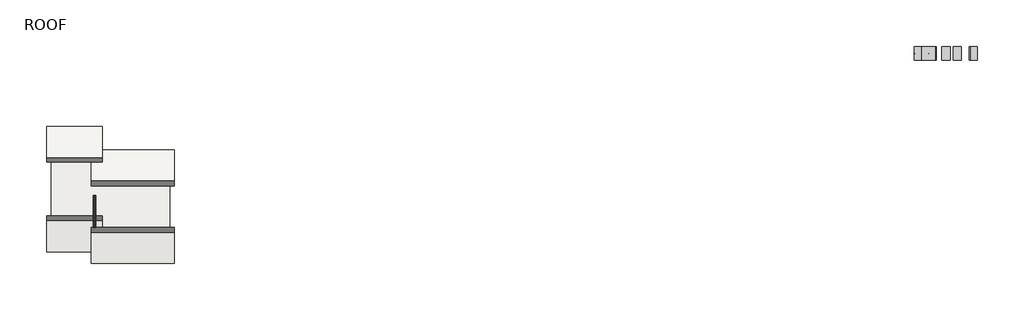
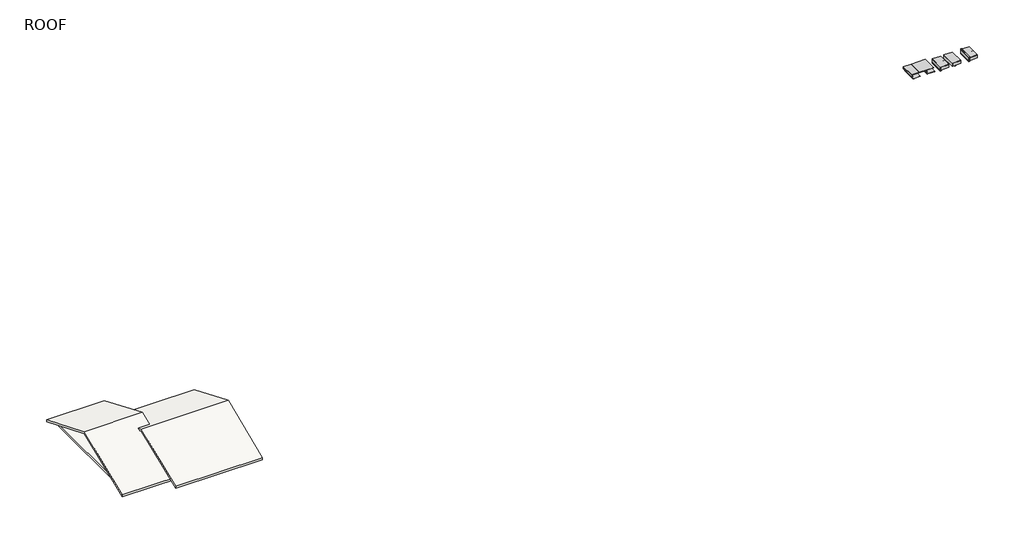
# One storey: 38 proxies, 2 roofs, 1 covering, 1 wall.
"""IFC4 building model written with IfcOpenShell, lengths in millimetres."""

import ifcopenshell
import ifcopenshell.guid

model = None  # the IFC model being written
_history = None  # IfcOwnerHistory: only IFC2X3 demands one
_inside = {}  # id of a spatial element -> (the spatial element, [elements in it])
_under = {}  # id of a project, library or spatial element -> (it, [spatial elements below it])
_declared = {}  # id of a project -> (the project, [libraries it declares])
_typed = {}  # id of a type object -> (the type object, [elements of that type])
_made_of = {}  # id of a material, layer set ... -> (it, [elements and type objects made of it])


def new_model(schema):
    """Start an empty IFC model of exactly this schema.

    Asked for "IFC4X3", IfcOpenShell would pick the latest addendum, in which some entities
    have other attributes; the version numbers below select the first issue.
    IFC2X3 requires an IfcOwnerHistory on every rooted entity: one is made here for all.
    """
    global model, _history
    if schema == "IFC4X3":
        model = ifcopenshell.file(schema_version=(4, 3, 0, 0))
    else:
        model = ifcopenshell.file(schema=schema)
    _inside.clear()
    _under.clear()
    _declared.clear()
    _typed.clear()
    _made_of.clear()
    _history = None
    if model.schema == "IFC2X3":
        org = make("IfcOrganization", Name="unknown")
        user = make(
            "IfcPersonAndOrganization",
            ThePerson=make("IfcPerson", FamilyName="unknown"),
            TheOrganization=org,
        )
        app = make(
            "IfcApplication",
            ApplicationDeveloper=org,
            Version="unknown",
            ApplicationFullName="unknown",
            ApplicationIdentifier="unknown",
        )
        _history = make(
            "IfcOwnerHistory",
            OwningUser=user,
            OwningApplication=app,
            ChangeAction="ADDED",
            CreationDate=0,
        )
    return model


def make(cls, **values):
    """One entity of the class cls with the attributes given. An attribute that is None is left unset."""
    return model.create_entity(
        cls, **{name: value for name, value in values.items() if value is not None}
    )


def rooted(cls, **values):
    """An entity with a GlobalId (a new one), such as an element, a storey or a relation."""
    return make(cls, GlobalId=ifcopenshell.guid.new(), OwnerHistory=_history, **values)


def si_unit(unit_type, name, prefix=None):
    """IfcSIUnit, for example si_unit("LENGTHUNIT", "METRE", prefix="MILLI")."""
    return make("IfcSIUnit", UnitType=unit_type, Prefix=prefix, Name=name)


def assignment(units):
    """IfcUnitAssignment: the units of a project."""
    return None if units is None else make("IfcUnitAssignment", Units=units)


def point(xyz):
    """IfcCartesianPoint."""
    return None if xyz is None else make("IfcCartesianPoint", Coordinates=xyz)


def direction(xyz):
    """IfcDirection."""
    return None if xyz is None else make("IfcDirection", DirectionRatios=xyz)


def frame(location, z_axis=None, x_axis=None):
    """IfcAxis2Placement3D, a coordinate frame: its origin and axes. An axis left out is left unset."""
    return make(
        "IfcAxis2Placement3D",
        Location=point(location),
        Axis=direction(z_axis),
        RefDirection=direction(x_axis),
    )


def origin():
    """The frame at (0, 0, 0) with its axes left unset."""
    return frame((0.0, 0.0, 0.0))


def place(relative_to, where):
    """IfcLocalPlacement: puts the frame where relative to a parent placement (None: the world)."""
    return make(
        "IfcLocalPlacement", PlacementRelTo=relative_to, RelativePlacement=where
    )


def context(
    kind, dimensions, precision=None, world=None, true_north=None, identifier=None
):
    """IfcGeometricRepresentationContext, for example the 3D "Model" context."""
    return make(
        "IfcGeometricRepresentationContext",
        ContextIdentifier=identifier,
        ContextType=kind,
        CoordinateSpaceDimension=dimensions,
        Precision=precision,
        WorldCoordinateSystem=world,
        TrueNorth=true_north,
    )


def project(units=None, contexts=None):
    """IfcProject with its units and contexts."""
    return rooted(
        "IfcProject",
        Name="project",
        RepresentationContexts=contexts,
        UnitsInContext=assignment(units),
    )


def spatial(cls, under=None, at=None, **own):
    """A site, building, storey or space (cls), placed at a placement, below another one or the project."""
    s = rooted(cls, ObjectPlacement=at, **own)
    if under is not None:
        _under.setdefault(under.id(), (under, []))[1].append(s)
    return s


def polyline(points):
    """IfcPolyline through the points."""
    return make("IfcPolyline", Points=[point(p) for p in points])


def outline(outer, holes=None, kind="AREA"):
    """IfcArbitraryClosedProfileDef: a profile drawn as a closed curve; with holes, ...WithVoids."""
    if holes is None:
        return make("IfcArbitraryClosedProfileDef", ProfileType=kind, OuterCurve=outer)
    return make(
        "IfcArbitraryProfileDefWithVoids",
        ProfileType=kind,
        OuterCurve=outer,
        InnerCurves=holes,
    )


def extrude(swept, where, along, depth):
    """IfcExtrudedAreaSolid: the profile swept, set in the frame where, extruded along a direction by depth."""
    return make(
        "IfcExtrudedAreaSolid",
        SweptArea=swept,
        Position=where,
        ExtrudedDirection=direction(along),
        Depth=depth,
    )


def faces_of(points, faces, orient=None, outer=None):
    """IfcFace entities. A face is a list of loops; a loop is a list of indices into points, from 0.

    orient and outer hold one flag for each loop. By default every Orientation is true, the
    first loop of a face is its IfcFaceOuterBound and the others are IfcFaceBound.
    """
    made = []
    for i, loops in enumerate(faces):
        bounds = []
        for j, loop in enumerate(loops):
            is_outer = j == 0 if outer is None else outer[i][j]
            bounds.append(
                make(
                    "IfcFaceOuterBound" if is_outer else "IfcFaceBound",
                    Bound=make("IfcPolyLoop", Polygon=[points[k] for k in loop]),
                    Orientation=True if orient is None else orient[i][j],
                )
            )
        made.append(make("IfcFace", Bounds=bounds))
    return made


def faceted_brep(points, faces, orient=None, outer=None, voids=None):
    """IfcFacetedBrep: a solid bounded by flat faces; with voids (closed shells), ...WithVoids."""
    shared = [point(p) for p in points]
    hull = make("IfcClosedShell", CfsFaces=faces_of(shared, faces, orient, outer))
    if voids is None:
        return make("IfcFacetedBrep", Outer=hull)
    return make(
        "IfcFacetedBrepWithVoids",
        Outer=hull,
        Voids=[
            make(cls, CfsFaces=faces_of(shared, fs, o, b)) for cls, fs, o, b in voids
        ],
    )


def shape(context_of_items, identifier, shape_type, items):
    """IfcShapeRepresentation: the items that make up one representation, for example the "Body"."""
    return make(
        "IfcShapeRepresentation",
        ContextOfItems=context_of_items,
        RepresentationIdentifier=identifier,
        RepresentationType=shape_type,
        Items=items,
    )


def source(mapping_origin, context_of_items, identifier, shape_type, items):
    """IfcRepresentationMap: a shape defined once, which mapped items show again and again."""
    return make(
        "IfcRepresentationMap",
        MappingOrigin=mapping_origin,
        MappedRepresentation=shape(context_of_items, identifier, shape_type, items),
    )


def transform(
    local_origin,
    x_axis=None,
    y_axis=None,
    z_axis=None,
    scale=None,
    scale2=None,
    scale3=None,
    uniform=True,
):
    """IfcCartesianTransformationOperator3D, or its non-uniform kind. x_axis, y_axis, z_axis: its Axis1, 2, 3."""
    if uniform:
        return make(
            "IfcCartesianTransformationOperator3D",
            Axis1=direction(x_axis),
            Axis2=direction(y_axis),
            LocalOrigin=point(local_origin),
            Scale=scale,
            Axis3=direction(z_axis),
        )
    return make(
        "IfcCartesianTransformationOperator3DnonUniform",
        Axis1=direction(x_axis),
        Axis2=direction(y_axis),
        LocalOrigin=point(local_origin),
        Scale=scale,
        Axis3=direction(z_axis),
        Scale2=scale2,
        Scale3=scale3,
    )


def mapped(mapping_source, mapping_target):
    """IfcMappedItem: shows the shape of a source again, moved by a transform."""
    return make(
        "IfcMappedItem", MappingSource=mapping_source, MappingTarget=mapping_target
    )


def made_of(thing, what):
    """Note that an element or type object is made of a material, layer set ...; save() writes the relation."""
    if what is not None:
        _made_of.setdefault(what.id(), (what, []))[1].append(thing)
    return thing


def element(
    cls,
    number,
    at=None,
    inside=None,
    cuts=None,
    type_object=None,
    material=None,
    context=None,
    identifier="Body",
    shape_type=None,
    held_by="IfcProductDefinitionShape",
    body=None,
    shapes=None,
    **own,
):
    """One element of the class cls, such as IfcWall. Its Tag is "e" and its number.

    at: its placement. inside: the storey or other place that contains it. cuts: it is an
    opening in that element (IfcRelVoidsElement). A single representation is given by context,
    identifier, shape_type and body (its items); several are given by shapes. held_by: the class
    of the entity that holds the representations. save() writes the other relations.
    """
    e = rooted(cls, Tag="e%d" % number, ObjectPlacement=at, **own)
    if body is not None:
        shapes = [shape(context, identifier, shape_type, body)]
    if shapes is not None:
        e.Representation = make(held_by, Representations=shapes)
    if inside is not None:
        _inside.setdefault(inside.id(), (inside, []))[1].append(e)
    if cuts is not None:
        rooted(
            "IfcRelVoidsElement", RelatingBuildingElement=cuts, RelatedOpeningElement=e
        )
    if type_object is not None:
        _typed.setdefault(type_object.id(), (type_object, []))[1].append(e)
    return made_of(e, material)


def aggregate(whole, parts):
    """IfcRelAggregates: a whole, such as a stair, and the parts it consists of."""
    return rooted("IfcRelAggregates", RelatingObject=whole, RelatedObjects=parts)


def save(model, path):
    """Write the relations noted so far, then the file.

    IfcRelAggregates (storeys below a building ...), IfcRelContainedInSpatialStructure (elements
    in a storey), IfcRelDefinesByType, IfcRelAssociatesMaterial and IfcRelDeclares: one each for
    every whole, place, type object, material and project.
    """
    for whole, parts in _under.values():
        aggregate(whole, parts)
    for where, things in _inside.values():
        rooted(
            "IfcRelContainedInSpatialStructure",
            RelatedElements=things,
            RelatingStructure=where,
        )
    for kind, things in _typed.values():
        rooted("IfcRelDefinesByType", RelatedObjects=things, RelatingType=kind)
    for what, things in _made_of.values():
        rooted("IfcRelAssociatesMaterial", RelatedObjects=things, RelatingMaterial=what)
    for by, libraries in _declared.values():
        rooted("IfcRelDeclares", RelatingContext=by, RelatedDefinitions=libraries)
    model.write(path)


def generic_models_10_generic_models_1_ea081297(model_context):
    return source(origin(), model_context, "Body", "SweptSolid", [
        extrude(outline(polyline([(49758.6, 0.0), (49720.5, 0.0), (49720.5, 1219.2), (49758.6, 1219.2), (49758.6, 0.0)])), frame((0.0, 0.0, 5507.83125), z_axis=(0.0, 0.0, 1.0), x_axis=(1.0, 0.0, 0.0)), (0.0, 0.0, 1.0), 139.7),
    ])


def generic_models_109_generic_models_1_8619d77b(model_context):
    return source(origin(), model_context, "Body", "SweptSolid", [
        extrude(outline(polyline([(51003.2, 0.0), (50914.3, 0.0), (50914.3, 1219.2), (51003.2, 1219.2), (51003.2, 0.0)])), frame((0.0, 0.0, 5184.378125), z_axis=(0.0, 0.0, 1.0), x_axis=(1.0, 0.0, 0.0)), (0.0, 0.0, 1.0), 38.1),
    ])


def generic_models_110_generic_models_1_6bdce9b6(model_context):
    return source(origin(), model_context, "Body", "SweptSolid", [
        extrude(outline(polyline([(51642.1451407, 1219.2), (51642.1451407, 0.0), (50914.3, 0.0), (50914.3, 1219.2), (51642.1451407, 1219.2)])), frame((0.0, 0.0, 5508.228125), z_axis=(0.0, 0.0, 1.0), x_axis=(1.0, 0.0, 0.0)), (0.0, 0.0, 1.0), 19.05),
    ])


def generic_models_112_generic_models_65_d168d7b0(model_context):
    return source(origin(), model_context, "Body", "SweptSolid", [
        extrude(outline(polyline([(50952.4, 592.1375), (50952.4, 630.2375), (51642.1451407, 630.2375), (51642.1451407, 592.1375), (50952.4, 592.1375)])), frame((0.0, 0.0, 5222.478125), z_axis=(0.0, 0.0, 1.0), x_axis=(1.0, 0.0, 0.0)), (0.0, 0.0, 1.0), 285.75),
    ])


def generic_models_113_generic_models_1_101608ab(model_context):
    return source(origin(), model_context, "Body", "SweptSolid", [
        extrude(outline(polyline([(52171.6, 0.0), (52133.5, 0.0), (52133.5, 1219.2), (52171.6, 1219.2), (52171.6, 0.0)])), frame((0.0, 0.0, 5222.478125), z_axis=(0.0, 0.0, 1.0), x_axis=(1.0, 0.0, 0.0)), (0.0, 0.0, 1.0), 285.75),
    ])


def generic_models_114_generic_models_1_a6fb1c2c(model_context):
    return source(origin(), model_context, "Body", "SweptSolid", [
        extrude(outline(polyline([(51642.1451407, 1219.2), (51642.1451407, 0.0), (50965.9242022, 0.0), (50965.9242022, 1219.2), (51642.1451407, 1219.2)])), frame((0.0, 0.0, 5237.6235034), z_axis=(0.0, 0.0, 1.0), x_axis=(1.0, 0.0, 0.0)), (0.0, 0.0, 1.0), 254.0),
    ])


def generic_models_12_generic_models_46_b8a9a4e8(model_context):
    return source(origin(), model_context, "Body", "SweptSolid", [
        extrude(outline(polyline([(49757.8505137, 0.0), (49721.1284797, 0.0), (49721.1284797, 1219.2), (49757.8505137, 1219.2), (49757.8505137, 0.0)])), frame((0.0, 0.0, 5505.7509163), z_axis=(0.0, 0.0, 1.0), x_axis=(1.0, 0.0, 0.0)), (0.0, 0.0, 1.0), 1.5875),
    ])


def generic_models_13_generic_models_65_9e643fb9(model_context):
    return source(origin(), model_context, "Body", "SweptSolid", [
        extrude(outline(polyline([(49128.3625, 592.1375), (49128.3625, 630.2375), (50347.5625, 630.2375), (50347.5625, 592.1375), (49128.3625, 592.1375)])), frame((0.0, 0.0, 5507.83125), z_axis=(0.0, 0.0, 1.0), x_axis=(1.0, 0.0, 0.0)), (0.0, 0.0, 1.0), 139.7),
    ])


def generic_models_14_generic_models_1_e8c90d4c(model_context):
    return source(origin(), model_context, "Body", "SweptSolid", [
        extrude(outline(polyline([(2277.1204978, 49799.875), (2239.0204978, 49799.875), (2239.0204978, 49825.275), (2240.6079978, 49825.275), (2240.6079978, 49801.4625), (2277.1204978, 49801.4625), (2277.1204978, 49799.875)])), frame((0.0, 0.0, 0.0), z_axis=(0.0, 1.0, 0.0), x_axis=(0.0, 0.0, 1.0)), (0.0, 0.0, 1.0), 1219.2),
    ])


def generic_models_22_generic_models_1_e5767157(model_context):
    return source(origin(), model_context, "Body", "SweptSolid", [
        extrude(outline(polyline([(2409.6091, 49800.66875), (2409.6091, 49799.875), (2407.0592364, 49799.875), (2405.4618473, 49749.075), (2404.6631527, 49749.075), (2403.0657636, 49799.875), (2400.5159, 49799.875), (2400.5159, 49800.66875), (2409.6091, 49800.66875)])), frame((0.0, 565.15, 0.0), z_axis=(0.0, 1.0, 0.0), x_axis=(0.0, 0.0, 1.0)), (0.0, 0.0, 1.0), 12.7),
    ])


def generic_models_226_generic_models_1_7dc37832(model_context):
    return source(origin(), model_context, "Body", "SweptSolid", [
        extrude(outline(polyline([(5263.35625, 49733.4159), (5263.35625, 49742.5091), (5264.15, 49742.5091), (5264.15, 49739.9592364), (5314.95, 49738.3618473), (5314.95, 49737.5631527), (5264.15, 49735.9657636), (5264.15, 49733.4159), (5263.35625, 49733.4159)])), frame((0.0, 565.15, 0.0), z_axis=(0.0, 1.0, 0.0), x_axis=(0.0, 0.0, 1.0)), (0.0, 0.0, 1.0), 12.7),
    ])


def generic_models_202_generic_models_1_0ad20a8b(model_context):
    return source(origin(), model_context, "Body", "SweptSolid", [
        extrude(outline(polyline([(2253.330428, 49813.3451407), (2242.217928, 49813.3451407), (2242.217928, 49826.0451407), (2234.280428, 49828.9341545), (2234.280428, 50422.9451407), (2253.330428, 50422.9451407), (2253.330428, 49813.3451407)])), frame((0.0, 0.0, 0.0), z_axis=(0.0, 1.0, 0.0), x_axis=(0.0, 0.0, 1.0)), (0.0, 0.0, 1.0), 1219.2),
    ])


def generic_models_233_generic_models_1_ae5bae41(model_context):
    return source(origin(), model_context, "Body", "SweptSolid", [
        extrude(outline(polyline([(48564.8, 0.0), (48475.9, 0.0), (48475.9, 1219.2), (48564.8, 1219.2), (48564.8, 0.0)])), frame((0.0, 0.0, 5467.35), z_axis=(0.0, 0.0, 1.0), x_axis=(1.0, 0.0, 0.0)), (0.0, 0.0, 1.0), 38.1),
    ])


def generic_models_236_generic_models_1_f8917e71(model_context):
    return source(origin(), model_context, "Body", "SweptSolid", [
        extrude(outline(polyline([(48507.65, 0.0), (48469.55, 0.0), (48469.55, 1219.2), (48507.65, 1219.2), (48507.65, 0.0)])), frame((0.0, 0.0, 5507.83125), z_axis=(0.0, 0.0, 1.0), x_axis=(1.0, 0.0, 0.0)), (0.0, 0.0, 1.0), 139.7),
    ])


def generic_models_237_generic_models_65_1df05f16(model_context):
    return source(origin(), model_context, "Body", "SweptSolid", [
        extrude(outline(polyline([(48469.55, 592.1375), (48469.55, 630.2375), (49128.3625, 630.2375), (49128.3625, 592.1375), (48469.55, 592.1375)])), frame((0.0, 0.0, 5507.83125), z_axis=(0.0, 0.0, 1.0), x_axis=(1.0, 0.0, 0.0)), (0.0, 0.0, 1.0), 139.7),
    ])


def generic_models_239_generic_models_46_95e6735a(model_context):
    return source(origin(), model_context, "Body", "SweptSolid", [
        extrude(outline(polyline([(50347.5625, 0.0), (49691.4320511, 0.0), (49691.4320511, 1219.2), (50347.5625, 1219.2), (50347.5625, 0.0)])), frame((0.0, 0.0, 5505.7509163), z_axis=(0.0, 0.0, 1.0), x_axis=(1.0, 0.0, 0.0)), (0.0, 0.0, 1.0), 1.5875),
    ])


def generic_models_240_generic_models_1_611786cf(model_context):
    return source(origin(), model_context, "Body", "SweptSolid", [
        extrude(outline(polyline([(49128.3625, 1219.2), (49128.3625, 0.0), (48469.55, 0.0), (48469.55, 1219.2), (49128.3625, 1219.2)])), frame((0.0, 0.0, 5649.9125), z_axis=(0.0, 0.0, 1.0), x_axis=(1.0, 0.0, 0.0)), (0.0, 0.0, 1.0), 19.05),
    ])


def generic_models_29_generic_models_1_59087225(model_context):
    return source(origin(), model_context, "Body", "SweptSolid", [
        extrude(outline(polyline([(50347.5625, 1219.2), (50347.5625, 0.0), (49128.3625, 0.0), (49128.3625, 1219.2), (50347.5625, 1219.2)])), frame((0.0, 0.0, 5647.53125), z_axis=(0.0, 0.0, 1.0), x_axis=(1.0, 0.0, 0.0)), (0.0, 0.0, 1.0), 19.05),
    ])


def generic_models_37_generic_models_1_916dd7c6(model_context):
    return source(origin(), model_context, "Body", "SweptSolid", [
        extrude(outline(polyline([(2409.6091, 49675.25625), (2400.5159, 49675.25625), (2400.5159, 49676.05), (2403.0657636, 49676.05), (2404.6631527, 49726.85), (2405.4618473, 49726.85), (2407.0592364, 49676.05), (2409.6091, 49676.05), (2409.6091, 49675.25625)])), frame((0.0, 565.15, 0.0), z_axis=(0.0, 1.0, 0.0), x_axis=(0.0, 0.0, 1.0)), (0.0, 0.0, 1.0), 12.7),
    ])


def generic_models_103_generic_models_1_250a6a11(model_context):
    return source(origin(), model_context, "Body", "SweptSolid", [
        extrude(outline(polyline([(49784.0, 0.0), (49695.1, 0.0), (49695.1, 1219.2), (49784.0, 1219.2), (49784.0, 0.0)])), frame((0.0, 0.0, 5264.15), z_axis=(0.0, 0.0, 1.0), x_axis=(1.0, 0.0, 0.0)), (0.0, 0.0, 1.0), 38.1),
    ])


def generic_models_71_generic_models_1_508a995f(model_context):
    return source(origin(), model_context, "Body", "SweptSolid", [
        extrude(outline(polyline([(50952.4, 0.0), (50914.3, 0.0), (50914.3, 1219.2), (50952.4, 1219.2), (50952.4, 0.0)])), frame((0.0, 0.0, 5222.478125), z_axis=(0.0, 0.0, 1.0), x_axis=(1.0, 0.0, 0.0)), (0.0, 0.0, 1.0), 285.75),
    ])


def generic_models_87_generic_models_1_55a64953(model_context):
    return source(origin(), model_context, "Body", "SweptSolid", [
        extrude(outline(polyline([(51968.4, 0.0), (51930.3, 0.0), (51930.3, 1219.2), (51968.4, 1219.2), (51968.4, 0.0)])), frame((0.0, 0.0, 5222.478125), z_axis=(0.0, 0.0, 1.0), x_axis=(1.0, 0.0, 0.0)), (0.0, 0.0, 1.0), 285.75),
    ])


model = new_model("IFC4")

# Units and contexts
model_context = context("Model", 3, world=origin())
ifc_project = project(units=[si_unit("LENGTHUNIT", "METRE", prefix="MILLI")], contexts=[model_context])

# Site, building, storey
site = spatial("IfcSite", under=ifc_project)
building = spatial("IfcBuilding", under=site)
storey = spatial("IfcBuildingStorey", under=building, Name="ROOF", Elevation=5130.8)

# Proxies
placement = place(None, origin())
generic_models_10_generic_models_1_shape = generic_models_10_generic_models_1_ea081297(model_context)
element("IfcBuildingElementProxy", 1, Name="Generic Models 10 : Generic Models 1", ObjectType="Generic Models 10 : Generic Models 1", at=placement, inside=storey, context=model_context, shape_type="MappedRepresentation", body=[
    mapped(generic_models_10_generic_models_1_shape, transform((0.0, 0.0, 0.0), x_axis=(1.0, 0.0, 0.0), y_axis=(0.0, 1.0, 0.0), z_axis=(0.0, 0.0, 1.0))),
])
generic_models_109_generic_models_1_shape = generic_models_109_generic_models_1_8619d77b(model_context)
element("IfcBuildingElementProxy", 2, Name="Generic Models 109 : Generic Models 1", ObjectType="Generic Models 109 : Generic Models 1", at=placement, inside=storey, context=model_context, shape_type="MappedRepresentation", body=[
    mapped(generic_models_109_generic_models_1_shape, transform((2438.4, 0.0, 0.0), x_axis=(1.0, 0.0, 0.0), y_axis=(0.0, 1.0, 0.0), z_axis=(0.0, 0.0, 1.0))),
])
generic_models_110_generic_models_1_shape = generic_models_110_generic_models_1_6bdce9b6(model_context)
element("IfcBuildingElementProxy", 3, Name="Generic Models 110 : Generic Models 1", ObjectType="Generic Models 110 : Generic Models 1", at=placement, inside=storey, context=model_context, shape_type="MappedRepresentation", body=[
    mapped(generic_models_110_generic_models_1_shape, transform((2438.4, 0.0, 0.0), x_axis=(1.0, 0.0, 0.0), y_axis=(0.0, 1.0, 0.0), z_axis=(0.0, 0.0, 1.0))),
])
element("IfcBuildingElementProxy", 4, Name="Generic Models 111 : Generic Models 1", ObjectType="Generic Models 111 : Generic Models 1", at=placement, inside=storey, context=model_context, shape_type="MappedRepresentation", body=[
    mapped(generic_models_109_generic_models_1_shape, transform((2438.4, 0.0, -38.1), x_axis=(1.0, 0.0, 0.0), y_axis=(0.0, 1.0, 0.0), z_axis=(0.0, 0.0, 1.0))),
])
generic_models_112_generic_models_65_shape = generic_models_112_generic_models_65_d168d7b0(model_context)
element("IfcBuildingElementProxy", 5, Name="Generic Models 112 : Generic Models 65", ObjectType="Generic Models 112 : Generic Models 65", at=placement, inside=storey, context=model_context, shape_type="MappedRepresentation", body=[
    mapped(generic_models_112_generic_models_65_shape, transform((2438.4, 0.0, 0.0), x_axis=(1.0, 0.0, 0.0), y_axis=(0.0, 1.0, 0.0), z_axis=(0.0, 0.0, 1.0))),
])
generic_models_113_generic_models_1_shape = generic_models_113_generic_models_1_101608ab(model_context)
element("IfcBuildingElementProxy", 6, Name="Generic Models 113 : Generic Models 1", ObjectType="Generic Models 113 : Generic Models 1", at=placement, inside=storey, context=model_context, shape_type="MappedRepresentation", body=[
    mapped(generic_models_113_generic_models_1_shape, transform((1219.2, 0.0, 0.0), x_axis=(1.0, 0.0, 0.0), y_axis=(0.0, 1.0, 0.0), z_axis=(0.0, 0.0, 1.0))),
])
generic_models_114_generic_models_1_shape = generic_models_114_generic_models_1_a6fb1c2c(model_context)
element("IfcBuildingElementProxy", 7, Name="Generic Models 114 : Generic Models 1", ObjectType="Generic Models 114 : Generic Models 1", at=placement, inside=storey, context=model_context, shape_type="MappedRepresentation", body=[
    mapped(generic_models_114_generic_models_1_shape, transform((2438.4, 0.0, 0.0), x_axis=(1.0, 0.0, 0.0), y_axis=(0.0, 1.0, 0.0), z_axis=(0.0, 0.0, 1.0))),
])
element("IfcBuildingElementProxy", 8, Name="Generic Models 115 : Generic Models 1", ObjectType="Generic Models 115 : Generic Models 1", at=placement, inside=storey, context=model_context, shape_type="MappedRepresentation", body=[
    mapped(generic_models_109_generic_models_1_shape, transform((2438.4, 0.0, 342.9), x_axis=(1.0, 0.0, 0.0), y_axis=(0.0, 1.0, 0.0), z_axis=(0.0, 0.0, 1.0))),
])
generic_models_12_generic_models_46_shape = generic_models_12_generic_models_46_b8a9a4e8(model_context)
element("IfcBuildingElementProxy", 9, Name="Generic Models 12 : Generic Models 46", ObjectType="Generic Models 12 : Generic Models 46", at=placement, inside=storey, context=model_context, shape_type="MappedRepresentation", body=[
    mapped(generic_models_12_generic_models_46_shape, transform((0.0, 0.0, 0.0), x_axis=(1.0, 0.0, 0.0), y_axis=(0.0, 1.0, 0.0), z_axis=(0.0, 0.0, 1.0))),
])
generic_models_13_generic_models_65_shape = generic_models_13_generic_models_65_9e643fb9(model_context)
element("IfcBuildingElementProxy", 10, Name="Generic Models 13 : Generic Models 65", ObjectType="Generic Models 13 : Generic Models 65", at=placement, inside=storey, context=model_context, shape_type="MappedRepresentation", body=[
    mapped(generic_models_13_generic_models_65_shape, transform((0.0, 0.0, 0.0), x_axis=(1.0, 0.0, 0.0), y_axis=(0.0, 1.0, 0.0), z_axis=(0.0, 0.0, 1.0))),
])
generic_models_14_generic_models_1_shape = generic_models_14_generic_models_1_e8c90d4c(model_context)
element("IfcBuildingElementProxy", 11, Name="Generic Models 14 : Generic Models 1", ObjectType="Generic Models 14 : Generic Models 1", at=placement, inside=storey, context=model_context, shape_type="MappedRepresentation", body=[
    mapped(generic_models_14_generic_models_1_shape, transform((0.0, 0.0, 3050.778125), x_axis=(1.0, 0.0, 0.0), y_axis=(0.0, 1.0, 0.0), z_axis=(0.0, 0.0, 1.0))),
])
generic_models_22_generic_models_1_shape = generic_models_22_generic_models_1_e5767157(model_context)
element("IfcBuildingElementProxy", 12, Name="Generic Models 22 : Generic Models 1", ObjectType="Generic Models 22 : Generic Models 1", at=placement, inside=storey, context=model_context, shape_type="MappedRepresentation", body=[
    mapped(generic_models_22_generic_models_1_shape, transform((0.0, 0.0, 3081.3375), x_axis=(1.0, 0.0, 0.0), y_axis=(0.0, 1.0, 0.0), z_axis=(0.0, 0.0, 1.0))),
])
element("IfcBuildingElementProxy", 13, Name="Generic Models 224 : Generic Models 1", ObjectType="Generic Models 224 : Generic Models 1", at=placement, inside=storey, context=model_context, shape_type="MappedRepresentation", body=[
    mapped(generic_models_14_generic_models_1_shape, transform((-1217.6125, 0.0, 3050.778125), x_axis=(1.0, 0.0, 0.0), y_axis=(0.0, 1.0, 0.0), z_axis=(0.0, 0.0, 1.0))),
])
element("IfcBuildingElementProxy", 14, Name="Generic Models 225 : Generic Models 1", ObjectType="Generic Models 225 : Generic Models 1", at=placement, inside=storey, context=model_context, shape_type="MappedRepresentation", body=[
    mapped(generic_models_22_generic_models_1_shape, transform((-1219.2, 0.0, 3081.3375), x_axis=(1.0, 0.0, 0.0), y_axis=(0.0, 1.0, 0.0), z_axis=(0.0, 0.0, 1.0))),
])
generic_models_226_generic_models_1_shape = generic_models_226_generic_models_1_7dc37832(model_context)
element("IfcBuildingElementProxy", 15, Name="Generic Models 226 : Generic Models 1", ObjectType="Generic Models 226 : Generic Models 1", at=placement, inside=storey, context=model_context, shape_type="MappedRepresentation", body=[
    mapped(generic_models_226_generic_models_1_shape, transform((-1219.2, 0.0, 203.2), x_axis=(1.0, 0.0, 0.0), y_axis=(0.0, 1.0, 0.0), z_axis=(0.0, 0.0, 1.0))),
])
generic_models_202_generic_models_1_shape = generic_models_202_generic_models_1_0ad20a8b(model_context)
element("IfcBuildingElementProxy", 16, Name="Generic Models 231 : Generic Models 1", ObjectType="Generic Models 231 : Generic Models 1", at=placement, inside=storey, context=model_context, shape_type="MappedRepresentation", body=[
    mapped(generic_models_202_generic_models_1_shape, transform((-1217.6125, 0.0, 3050.778125), x_axis=(1.0, 0.0, 0.0), y_axis=(0.0, 1.0, 0.0), z_axis=(0.0, 0.0, 1.0))),
])
generic_models_233_generic_models_1_shape = generic_models_233_generic_models_1_ae5bae41(model_context)
element("IfcBuildingElementProxy", 17, Name="Generic Models 233 : Generic Models 1", ObjectType="Generic Models 233 : Generic Models 1", at=placement, inside=storey, context=model_context, shape_type="MappedRepresentation", body=[
    mapped(generic_models_233_generic_models_1_shape, transform((0.0, 0.0, 0.0), x_axis=(1.0, 0.0, 0.0), y_axis=(0.0, 1.0, 0.0), z_axis=(0.0, 0.0, 1.0))),
])
generic_models_236_generic_models_1_shape = generic_models_236_generic_models_1_f8917e71(model_context)
element("IfcBuildingElementProxy", 18, Name="Generic Models 236 : Generic Models 1", ObjectType="Generic Models 236 : Generic Models 1", at=placement, inside=storey, context=model_context, shape_type="MappedRepresentation", body=[
    mapped(generic_models_236_generic_models_1_shape, transform((0.0, 0.0, 0.0), x_axis=(1.0, 0.0, 0.0), y_axis=(0.0, 1.0, 0.0), z_axis=(0.0, 0.0, 1.0))),
])
generic_models_237_generic_models_65_shape = generic_models_237_generic_models_65_1df05f16(model_context)
element("IfcBuildingElementProxy", 19, Name="Generic Models 237 : Generic Models 65", ObjectType="Generic Models 237 : Generic Models 65", at=placement, inside=storey, context=model_context, shape_type="MappedRepresentation", body=[
    mapped(generic_models_237_generic_models_65_shape, transform((0.0, 0.0, 0.0), x_axis=(1.0, 0.0, 0.0), y_axis=(0.0, 1.0, 0.0), z_axis=(0.0, 0.0, 1.0))),
])
generic_models_239_generic_models_46_shape = generic_models_239_generic_models_46_95e6735a(model_context)
element("IfcBuildingElementProxy", 20, Name="Generic Models 239 : Generic Models 46", ObjectType="Generic Models 239 : Generic Models 46", at=placement, inside=storey, context=model_context, shape_type="MappedRepresentation", body=[
    mapped(generic_models_239_generic_models_46_shape, transform((-1219.2, 0.0, 142.08125), x_axis=(1.0, 0.0, 0.0), y_axis=(0.0, 1.0, 0.0), z_axis=(0.0, 0.0, 1.0))),
])
generic_models_240_generic_models_1_shape = generic_models_240_generic_models_1_611786cf(model_context)
element("IfcBuildingElementProxy", 21, Name="Generic Models 240 : Generic Models 1", ObjectType="Generic Models 240 : Generic Models 1", at=placement, inside=storey, context=model_context, shape_type="MappedRepresentation", body=[
    mapped(generic_models_240_generic_models_1_shape, transform((0.0, 0.0, 0.0), x_axis=(1.0, 0.0, 0.0), y_axis=(0.0, 1.0, 0.0), z_axis=(0.0, 0.0, 1.0))),
])
element("IfcBuildingElementProxy", 22, Name="Generic Models 25 : Generic Models 46", ObjectType="Generic Models 25 : Generic Models 46", at=placement, inside=storey, context=model_context, shape_type="MappedRepresentation", body=[
    mapped(generic_models_12_generic_models_46_shape, transform((0.0, 0.0, 142.08125), x_axis=(1.0, 0.0, 0.0), y_axis=(0.0, 1.0, 0.0), z_axis=(0.0, 0.0, 1.0))),
])
generic_models_29_generic_models_1_shape = generic_models_29_generic_models_1_59087225(model_context)
element("IfcBuildingElementProxy", 23, Name="Generic Models 29 : Generic Models 1", ObjectType="Generic Models 29 : Generic Models 1", at=placement, inside=storey, context=model_context, shape_type="MappedRepresentation", body=[
    mapped(generic_models_29_generic_models_1_shape, transform((0.0, 0.0, 2.38125), x_axis=(1.0, 0.0, 0.0), y_axis=(0.0, 1.0, 0.0), z_axis=(0.0, 0.0, 1.0))),
])
element("IfcBuildingElementProxy", 24, Name="Generic Models 39 : Generic Models 1", ObjectType="Generic Models 39 : Generic Models 1", at=placement, inside=storey, context=model_context, shape_type="MappedRepresentation", body=[
    mapped(generic_models_226_generic_models_1_shape, transform((0.0, 0.0, 203.2), x_axis=(1.0, 0.0, 0.0), y_axis=(0.0, 1.0, 0.0), z_axis=(0.0, 0.0, 1.0))),
])
generic_models_37_generic_models_1_shape = generic_models_37_generic_models_1_916dd7c6(model_context)
element("IfcBuildingElementProxy", 25, Name="Generic Models 47 : Generic Models 1", ObjectType="Generic Models 47 : Generic Models 1", at=placement, inside=storey, context=model_context, shape_type="MappedRepresentation", body=[
    mapped(generic_models_37_generic_models_1_shape, transform((3.175, 0.0, 3081.3375), x_axis=(1.0, 0.0, 0.0), y_axis=(0.0, 1.0, 0.0), z_axis=(0.0, 0.0, 1.0))),
])
element("IfcBuildingElementProxy", 26, Name="Generic Models 49 : Generic Models 1", ObjectType="Generic Models 49 : Generic Models 1", at=placement, inside=storey, context=model_context, shape_type="MappedRepresentation", body=[
    mapped(generic_models_202_generic_models_1_shape, transform((0.0, 0.0, 3050.778125), x_axis=(1.0, 0.0, 0.0), y_axis=(0.0, 1.0, 0.0), z_axis=(0.0, 0.0, 1.0))),
])
element("IfcBuildingElementProxy", 27, Name="Generic Models 59 : Generic Models 65", ObjectType="Generic Models 59 : Generic Models 65", at=placement, inside=storey, context=model_context, shape_type="MappedRepresentation", body=[
    mapped(generic_models_112_generic_models_65_shape, transform((0.0, 0.0, 0.0), x_axis=(1.0, 0.0, 0.0), y_axis=(0.0, 1.0, 0.0), z_axis=(0.0, 0.0, 1.0))),
])
generic_models_103_generic_models_1_shape = generic_models_103_generic_models_1_250a6a11(model_context)
element("IfcBuildingElementProxy", 28, Name="Generic Models 6 : Generic Models 1", ObjectType="Generic Models 6 : Generic Models 1", at=placement, inside=storey, context=model_context, shape_type="MappedRepresentation", body=[
    mapped(generic_models_103_generic_models_1_shape, transform((0.0, 0.0, 203.2), x_axis=(1.0, 0.0, 0.0), y_axis=(0.0, 1.0, 0.0), z_axis=(0.0, 0.0, 1.0))),
])
element("IfcBuildingElementProxy", 29, Name="Generic Models 64 : Generic Models 1", ObjectType="Generic Models 64 : Generic Models 1", at=placement, inside=storey, context=model_context, shape_type="MappedRepresentation", body=[
    mapped(generic_models_109_generic_models_1_shape, transform((0.0, 0.0, 0.0), x_axis=(1.0, 0.0, 0.0), y_axis=(0.0, 1.0, 0.0), z_axis=(0.0, 0.0, 1.0))),
])
element("IfcBuildingElementProxy", 30, Name="Generic Models 66 : Generic Models 1", ObjectType="Generic Models 66 : Generic Models 1", at=placement, inside=storey, context=model_context, shape_type="MappedRepresentation", body=[
    mapped(generic_models_110_generic_models_1_shape, transform((0.0, 0.0, 0.0), x_axis=(1.0, 0.0, 0.0), y_axis=(0.0, 1.0, 0.0), z_axis=(0.0, 0.0, 1.0))),
])
element("IfcBuildingElementProxy", 31, Name="Generic Models 70 : Generic Models 1", ObjectType="Generic Models 70 : Generic Models 1", at=placement, inside=storey, context=model_context, shape_type="MappedRepresentation", body=[
    mapped(generic_models_109_generic_models_1_shape, transform((0.0, 0.0, -38.1), x_axis=(1.0, 0.0, 0.0), y_axis=(0.0, 1.0, 0.0), z_axis=(0.0, 0.0, 1.0))),
])
generic_models_71_generic_models_1_shape = generic_models_71_generic_models_1_508a995f(model_context)
element("IfcBuildingElementProxy", 32, Name="Generic Models 71 : Generic Models 1", ObjectType="Generic Models 71 : Generic Models 1", at=placement, inside=storey, context=model_context, shape_type="MappedRepresentation", body=[
    mapped(generic_models_71_generic_models_1_shape, transform((0.0, 0.0, 0.0), x_axis=(1.0, 0.0, 0.0), y_axis=(0.0, 1.0, 0.0), z_axis=(0.0, 0.0, 1.0))),
])
element("IfcBuildingElementProxy", 33, Name="Generic Models 72 : Generic Models 1", ObjectType="Generic Models 72 : Generic Models 1", at=placement, inside=storey, context=model_context, shape_type="MappedRepresentation", body=[
    mapped(generic_models_114_generic_models_1_shape, transform((0.0, 0.0, 0.0), x_axis=(1.0, 0.0, 0.0), y_axis=(0.0, 1.0, 0.0), z_axis=(0.0, 0.0, 1.0))),
])
element("IfcBuildingElementProxy", 34, Name="Generic Models 81 : Generic Models 1", ObjectType="Generic Models 81 : Generic Models 1", at=placement, inside=storey, context=model_context, shape_type="MappedRepresentation", body=[
    mapped(generic_models_109_generic_models_1_shape, transform((1219.2, 0.0, 0.0), x_axis=(1.0, 0.0, 0.0), y_axis=(0.0, 1.0, 0.0), z_axis=(0.0, 0.0, 1.0))),
])
element("IfcBuildingElementProxy", 35, Name="Generic Models 82 : Generic Models 1", ObjectType="Generic Models 82 : Generic Models 1", at=placement, inside=storey, context=model_context, shape_type="MappedRepresentation", body=[
    mapped(generic_models_110_generic_models_1_shape, transform((1016.0, 0.0, 0.0), x_axis=(1.0, 0.0, 0.0), y_axis=(0.0, 1.0, 0.0), z_axis=(0.0, 0.0, 1.0))),
])
element("IfcBuildingElementProxy", 36, Name="Generic Models 86 : Generic Models 65", ObjectType="Generic Models 86 : Generic Models 65", at=placement, inside=storey, context=model_context, shape_type="MappedRepresentation", body=[
    mapped(generic_models_112_generic_models_65_shape, transform((1016.0, 0.0, 0.0), x_axis=(1.0, 0.0, 0.0), y_axis=(0.0, 1.0, 0.0), z_axis=(0.0, 0.0, 1.0))),
])
generic_models_87_generic_models_1_shape = generic_models_87_generic_models_1_55a64953(model_context)
element("IfcBuildingElementProxy", 37, Name="Generic Models 87 : Generic Models 1", ObjectType="Generic Models 87 : Generic Models 1", at=placement, inside=storey, context=model_context, shape_type="MappedRepresentation", body=[
    mapped(generic_models_87_generic_models_1_shape, transform((0.0, 0.0, 0.0), x_axis=(1.0, 0.0, 0.0), y_axis=(0.0, 1.0, 0.0), z_axis=(0.0, 0.0, 1.0))),
])
element("IfcBuildingElementProxy", 38, Name="Generic Models 88 : Generic Models 1", ObjectType="Generic Models 88 : Generic Models 1", at=placement, inside=storey, context=model_context, shape_type="MappedRepresentation", body=[
    mapped(generic_models_114_generic_models_1_shape, transform((1016.0, 0.0, 0.0), x_axis=(1.0, 0.0, 0.0), y_axis=(0.0, 1.0, 0.0), z_axis=(0.0, 0.0, 1.0))),
])

# Covering
element("IfcCovering", 39, ObjectType="GYP. BD WITH INSULATION", at=placement, inside=storey, context=model_context, shape_type="Brep", body=[
    faceted_brep([(-28217.4664763, -16236.2070712, 5311.775), (-24255.0664763, -16236.2070712, 5311.775), (-24255.0664763, -16325.7420712, 5311.775), (-24255.0664763, -17335.3920712, 5311.775), (-17689.1664763, -17335.3920712, 5311.775), (-17689.1664763, -8742.5720712, 5311.775), (-24664.6414763, -8742.5720712, 5311.775), (-24664.6414763, -8313.3120712, 5311.775), (-24102.6664763, -8313.3120712, 5311.775), (-24102.6664763, -6304.8070712, 5311.775), (-28217.4664763, -6304.8070712, 5311.775), (-24255.0664763, -16236.2070712, 5130.8), (-28217.4664763, -16236.2070712, 5130.8), (-28217.4664763, -6304.8070712, 5130.8), (-24102.6664763, -6304.8070712, 5130.8), (-24102.6664763, -8003.4320712, 5130.8), (-24664.6414763, -8003.4320712, 5130.8), (-24664.6414763, -8308.2320712, 5130.8), (-24102.6664763, -8308.2320712, 5130.8), (-24102.6664763, -8413.0070712, 5130.8), (-17689.1664763, -8413.0070712, 5130.8), (-17689.1664763, -17664.9570712, 5130.8), (-24255.0664763, -17664.9570712, 5130.8), (-24255.0664763, -16445.7570712, 5130.8), (-24255.0664763, -17664.9570712, 5174.45625), (-17689.1664763, -17664.9570712, 5174.45625), (-17689.1664763, -8413.0070712, 5174.45625), (-24102.6664763, -8413.0070712, 5174.45625), (-24102.6664763, -8003.4320712, 5182.6583333), (-24664.6414763, -8003.4320712, 5182.6583333)], [[[0, 1, 2, 3, 4, 5, 6, 7, 8, 9, 10]], [[11, 12, 13, 14, 15, 16, 17, 18, 19, 20, 21, 22, 23]], [[1, 0, 12, 11]], [[11, 23, 22, 24, 3, 2, 1]], [[22, 21, 25, 24]], [[21, 20, 26, 5, 4, 25]], [[20, 19, 27, 26]], [[14, 9, 8, 28, 15]], [[19, 18, 27]], [[10, 9, 14, 13]], [[0, 10, 13, 12]], [[17, 6, 5, 26, 27, 18]], [[4, 3, 24, 25]], [[7, 29, 28, 8]], [[28, 29, 16, 15]], [[6, 17, 16, 29, 7]]]),
])

# Roofs
element("IfcRoof", 40, ObjectType="Generic - 6 1/2\"", at=placement, inside=storey, context=model_context, shape_type="SweptSolid", body=[
    extrude(outline(polyline([(-17064.8820712, 5182.6583333), (-11480.0570712, 7509.66875), (-5895.2320712, 5182.6583333), (-5895.2320712, 5003.8), (-11480.0570712, 7330.8104167), (-17064.8820712, 5003.8), (-17064.8820712, 5182.6583333)])), frame((-28627.0414763, 0.0, 0.0), z_axis=(1.0, 0.0, 0.0), x_axis=(0.0, 1.0, 0.0)), (0.0, 0.0, 1.0), 4933.95),
])
element("IfcRoof", 41, ObjectType="Generic - 6 1/2\"", at=placement, inside=storey, context=model_context, shape_type="Brep", body=[
    faceted_brep([(-24664.6414763, -8003.4320712, 5003.8), (-17279.5914763, -8003.4320712, 5003.8), (-17279.5914763, -13038.9820712, 7101.9458333), (-24664.6414763, -13038.9820712, 7101.9458333), (-24664.6414763, -8742.5720712, 5311.775), (-24664.6414763, -8308.2320712, 5130.8), (-17279.5914763, -18074.5320712, 5003.8), (-24664.6414763, -18074.5320712, 5003.8), (-17279.5914763, -8003.4320712, 5182.6583333), (-24102.6664763, -8003.4320712, 5182.6583333), (-24664.6414763, -8003.4320712, 5182.6583333), (-24664.6414763, -8313.3120712, 5311.775), (-24664.6414763, -13038.9820712, 7280.8041667), (-17279.5914763, -13038.9820712, 7280.8041667), (-17279.5914763, -18074.5320712, 5182.6583333), (-24664.6414763, -18074.5320712, 5182.6583333), (-24664.6414763, -8003.4320712, 5130.8)], [[[0, 1, 2, 3, 4, 5]], [[2, 6, 7, 3]], [[8, 9, 10, 11, 12, 13]], [[14, 13, 12, 15]], [[0, 16, 10, 9, 8, 1]], [[6, 14, 15, 7]], [[8, 13, 14, 6, 2, 1]], [[15, 12, 11, 10, 16, 0, 5, 4, 3, 7]]]),
])

# Wall
element("IfcWall", 42, ObjectType="Upper Wall", at=placement, inside=storey, context=model_context, shape_type="SweptSolid", body=[
    extrude(outline(polyline([(-12035.6820712, 5130.8), (-16655.3070712, 5130.8), (-16655.3070712, 5174.45625), (-16744.2070712, 5174.45625), (-16744.2070712, 5558.1020833), (-13038.9820712, 7101.9458333), (-12035.6820712, 6683.9041667), (-12035.6820712, 5130.8)])), frame((-24464.6164763, 0.0, 0.0), z_axis=(1.0, 0.0, 0.0), x_axis=(0.0, 1.0, 0.0)), (0.0, 0.0, 1.0), 209.55),
])

save(model, "model.ifc")

# Revit data of these elements
# Project information
#   Project Issue Date = "09/11/2018"
#   Project Status = "Project Status"
#   Client Name = "Owner"
#   Project Address = "1021 HIGH ST -  MADISON, WI 53715"
#   Project Name = "2ND FLOOR ADDITION"
#   Project Number = "Project Number"
# Grids (mm)
#   "B": line (-20559.366, -20481.133) -> (-20559.366, -4657.508)
#   "C": line (-23277.166, -20481.133) -> (-23277.166, -4657.508)
#   "D": line (-25994.966, -20481.133) -> (-25994.966, -4657.508)
# Type "GYP. BD WITH INSULATION"
#   Assembly Code = "C3030220"
#   built-in parameter 1002203 = 1 (stored number, unit not read)
#   built-in parameter 1002202 = 1 (stored number, unit not read)
#   Layers, outside or top first: 0' - 6 1/2" "R49 BATT INSULATION AT CEILING JOISTS - VENTS AT EAVES AND RIDGE" (function 1); 0' - 0 5/8" "5/8\" GYP. BD" (function 5)
# Type "Generic - 6 1/2\""
#   Assembly Code = "B1020"
#   Layers, outside or top first: 0' - 0 1/4" "ASPHALT SHINGLES" (function 1); 0' - 0 3/4" "30 LB. BUILDINGS FELT OVER 3/4\" CDX PLYWOOD" (function 1); 0' - 5 1/2" "PRE-ENGINEERED TRUSSES" (function 1)
# Type "Upper Wall"
#   Assembly Code = "B2010"
#   Fire_Rating = "2 HR"
#   Layers, outside or top first: 0' - 0 1/4" "Upper Finish" (function 5); 0' - 1 1/2" "1 1/2\" RIGID FOAM" (function 3); 0' - 0 1/2" "1/2\" CDX PLYWOOD" (function 2); 0' - 5 1/2" "2X6 INSULATED WALL CAVITY" (function 1); 0' - 0 1/2" "1/2\" GYP. BD OVER VAPOR BARRIER" (function 5)
# Element 1 (IfcBuildingElementProxy, "Generic Models 10 : Generic Models 1")
#   Phase Created = _ZAVE
#   Materials on its faces: "2X BLOCKING - LOCATED AT GRAB BARS, WALL HUNG CABINETS, ETC.)"
# Element 2 (IfcBuildingElementProxy, "Generic Models 109 : Generic Models 1")
#   Phase Created = _ZAVE
#   Materials on its faces: "DOUBLE 2X WOOD TOP PLATE"
# Element 3 (IfcBuildingElementProxy, "Generic Models 110 : Generic Models 1")
#   Phase Created = _ZAVE
#   Materials on its faces: "3/4\" CDX PLYWOOD"
# Element 4 (IfcBuildingElementProxy, "Generic Models 111 : Generic Models 1")
#   Phase Created = _ZAVE
#   Materials on its faces: "DOUBLE 2X WOOD TOP PLATE"
# Element 5 (IfcBuildingElementProxy, "Generic Models 112 : Generic Models 65")
#   Phase Created = _ZAVE
#   Materials on its faces: "WOOD JOIST AS SPECIFIED"
# Element 6 (IfcBuildingElementProxy, "Generic Models 113 : Generic Models 1")
#   Phase Created = _ZAVE
#   Materials on its faces: "RIM BOARD - SIZE TO MATCH JOIST DEPTH"
# Element 7 (IfcBuildingElementProxy, "Generic Models 114 : Generic Models 1")
#   Phase Created = _ZAVE
#   Materials on its faces: "SOUND BATT. INSULATION"
# Element 8 (IfcBuildingElementProxy, "Generic Models 115 : Generic Models 1")
#   Phase Created = _ZAVE
#   Materials on its faces: "DOUBLE 2X WOOD TOP PLATE"
# Element 9 (IfcBuildingElementProxy, "Generic Models 12 : Generic Models 46")
#   Phase Created = _ZAVE
#   Materials on its faces: "SET IN BED OF SEALANT"
# Element 10 (IfcBuildingElementProxy, "Generic Models 13 : Generic Models 65")
#   Phase Created = _ZAVE
#   Materials on its faces: "WOOD JOIST AS SPECIFIED"
# Element 11 (IfcBuildingElementProxy, "Generic Models 14 : Generic Models 1")
#   Phase Created = _ZAVE
#   Materials on its faces: "CEILING TRACK AS SCHEDULED"
# Element 12 (IfcBuildingElementProxy, "Generic Models 22 : Generic Models 1")
#   Phase Created = _ZAVE
#   Materials on its faces: "ATTACH GYPSUM BOARD TO STUDS AND NOT TO TOP TRACK"
# Element 13 (IfcBuildingElementProxy, "Generic Models 224 : Generic Models 1")
#   Phase Created = _ZAVE
#   Materials on its faces: "CEILING TRACK AS SCHEDULED"
# Element 14 (IfcBuildingElementProxy, "Generic Models 225 : Generic Models 1")
#   Phase Created = _ZAVE
#   Materials on its faces: "ATTACH GYPSUM BOARD TO STUDS AND NOT TO TOP TRACK"
# Element 15 (IfcBuildingElementProxy, "Generic Models 226 : Generic Models 1")
#   Phase Created = _ZAVE
#   Materials on its faces: "METAL RUNNER CHANNEL; FASTEN @ 24\" O.C."
# Element 16 (IfcBuildingElementProxy, "Generic Models 231 : Generic Models 1")
#   Phase Created = _ZAVE
#   Materials on its faces: "CEILING AS SCHEDULED"
# Element 17 (IfcBuildingElementProxy, "Generic Models 233 : Generic Models 1")
#   Phase Created = _ZAVE
#   Materials on its faces: "2X WOOD HEADER ATTACHED TO STEEL PURLIN"
# Element 18 (IfcBuildingElementProxy, "Generic Models 236 : Generic Models 1")
#   Phase Created = _ZAVE
#   Materials on its faces: "EXISTING RIM BOARD OR JOIST"
# Element 19 (IfcBuildingElementProxy, "Generic Models 237 : Generic Models 65")
#   Phase Created = _ZAVE
#   Materials on its faces: "WOOD JOIST AS SPECIFIED"
# Element 20 (IfcBuildingElementProxy, "Generic Models 239 : Generic Models 46")
#   Phase Created = _ZAVE
#   Materials on its faces: "SET IN BED OF SEALANT"
# Element 21 (IfcBuildingElementProxy, "Generic Models 240 : Generic Models 1")
#   Phase Created = _ZAVE
#   Materials on its faces: "EXISTING SUBSTRATE"
# Element 22 (IfcBuildingElementProxy, "Generic Models 25 : Generic Models 46")
#   Phase Created = _ZAVE
#   Materials on its faces: "SET IN BED OF SEALANT"
# Element 23 (IfcBuildingElementProxy, "Generic Models 29 : Generic Models 1")
#   Phase Created = _ZAVE
#   Materials on its faces: "SUBSTRATE AS SCHEDULED"
# Element 24 (IfcBuildingElementProxy, "Generic Models 39 : Generic Models 1")
#   Phase Created = _ZAVE
#   Materials on its faces: "METAL RUNNER CHANNEL; FASTEN @ 24\" O.C."
# Element 25 (IfcBuildingElementProxy, "Generic Models 47 : Generic Models 1")
#   Phase Created = _ZAVE
#   Materials on its faces: "ATTACH GYPSUM BOARD TO STUDS AND NOT TO TOP TRACK"
# Element 26 (IfcBuildingElementProxy, "Generic Models 49 : Generic Models 1")
#   Phase Created = _ZAVE
#   Materials on its faces: "CEILING AS SCHEDULED"
# Element 27 (IfcBuildingElementProxy, "Generic Models 59 : Generic Models 65")
#   Phase Created = _ZAVE
#   Materials on its faces: "WOOD JOIST AS SPECIFIED"
# Element 28 (IfcBuildingElementProxy, "Generic Models 6 : Generic Models 1")
#   Phase Created = _ZAVE
#   Materials on its faces: "2X WOOD HEADER ATTACHED TO STEEL PURLIN"
# Element 29 (IfcBuildingElementProxy, "Generic Models 64 : Generic Models 1")
#   Phase Created = _ZAVE
#   Materials on its faces: "DOUBLE 2X WOOD TOP PLATE"
# Element 30 (IfcBuildingElementProxy, "Generic Models 66 : Generic Models 1")
#   Phase Created = _ZAVE
#   Materials on its faces: "3/4\" CDX PLYWOOD"
# Element 31 (IfcBuildingElementProxy, "Generic Models 70 : Generic Models 1")
#   Phase Created = _ZAVE
#   Materials on its faces: "DOUBLE 2X WOOD TOP PLATE"
# Element 32 (IfcBuildingElementProxy, "Generic Models 71 : Generic Models 1")
#   Phase Created = _ZAVE
#   Materials on its faces: "DOUBLE 2X WOOD TOP PLATE"
# Element 33 (IfcBuildingElementProxy, "Generic Models 72 : Generic Models 1")
#   Phase Created = _ZAVE
#   Materials on its faces: "SOUND BATT. INSULATION"
# Element 34 (IfcBuildingElementProxy, "Generic Models 81 : Generic Models 1")
#   Phase Created = _ZAVE
#   Materials on its faces: "DOUBLE 2X WOOD TOP PLATE"
# Element 35 (IfcBuildingElementProxy, "Generic Models 82 : Generic Models 1")
#   Phase Created = _ZAVE
#   Materials on its faces: "3/4\" CDX PLYWOOD"
# Element 36 (IfcBuildingElementProxy, "Generic Models 86 : Generic Models 65")
#   Phase Created = _ZAVE
#   Materials on its faces: "WOOD JOIST AS SPECIFIED"
# Element 37 (IfcBuildingElementProxy, "Generic Models 87 : Generic Models 1")
#   Phase Created = _ZAVE
#   Materials on its faces: "2X12 LEDGER WITH HILTI 3/8* DIAMETER HLC SLEEVE ANCHOR @ 8” OC."
# Element 38 (IfcBuildingElementProxy, "Generic Models 88 : Generic Models 1")
#   Phase Created = _ZAVE
#   Materials on its faces: "SOUND BATT. INSULATION"
# Element 39 (IfcCovering, "GYP. BD WITH INSULATION")
#   Height Offset From Level = 0' - 0"
#   Phase Created = 1st Phase
#   Materials on its faces: "5/8\" GYP. BD", "R49 BATT INSULATION AT CEILING JOISTS - VENTS AT EAVES AND RIDGE"
# Element 40 (IfcRoof, "Generic - 6 1/2\"")
#   built-in parameter 1001705 = 24.638 (stored number, unit not read)
#   built-in parameter 1001710 = 33615
#   Phase Created = 1st Phase
#   Materials on its faces: "PRE-ENGINEERED TRUSSES", "ASPHALT SHINGLES"
# Element 41 (IfcRoof, "Generic - 6 1/2\"")
#   built-in parameter 1001705 = 23.8872 (stored number, unit not read)
#   built-in parameter 1001710 = 33615
#   Phase Created = 1st Phase
#   Materials on its faces: "PRE-ENGINEERED TRUSSES", "ASPHALT SHINGLES"
# Element 42 (IfcWall, "Upper Wall")
#   Top Offset = 8' - 8.49189"
#   Base Offset = 0' - 0"
#   wall height = 8' - 8.49189"
#   Phase Created = 1st Phase
#   Base Constraint = ROOF
#   Top Constraint = ROOF
#   Materials on its faces: "Upper Finish", "1/2\" GYP. BD OVER VAPOR BARRIER"
# Materials
#   "R49 BATT INSULATION AT CEILING JOISTS - VENTS AT EAVES AND RIDGE": class "Wood", colour RGB 234 198 147, transparency 0, Description = "Pinus Echinata", Cost = 0
#   "5/8\" GYP. BD": class "Generic", colour RGB 255 255 255, transparency 0, Description = "Gypsum Wall Board", Cost = 0
#   "ASPHALT SHINGLES": class "Generic", colour RGB 105 104 104, transparency 0, Description = "Asphalt roofing shingle", Cost = 0
#   "30 LB. BUILDINGS FELT OVER 3/4\" CDX PLYWOOD": class "Unassigned", colour RGB 196 177 123, transparency 0, Cost = 0
#   "PRE-ENGINEERED TRUSSES": class "Wood", colour RGB 234 198 147, transparency 0, Description = "Pinus Echinata", Cost = 0
#   "Upper Finish": class "Generic", colour RGB 190 190 124, transparency 0, Cost = 0
#   "1 1/2\" RIGID FOAM": class "Miscellaneous", colour RGB 98 154 157, transparency 0, Cost = 0
#   "1/2\" CDX PLYWOOD": class "Unassigned", colour RGB 196 177 123, transparency 0, Cost = 0
#   "2X6 INSULATED WALL CAVITY": class "Wood", colour RGB 234 198 147, transparency 0, Description = "Pinus Echinata", Cost = 0
#   "1/2\" GYP. BD OVER VAPOR BARRIER": class "Generic", colour RGB 255 255 255, transparency 0, Description = "Gypsum Wall Board", Cost = 0
#   "2X BLOCKING - LOCATED AT GRAB BARS, WALL HUNG CABINETS, ETC.)": class "Wood", colour RGB 234 198 147, transparency 0, Description = "Pinus Echinata", Cost = 0
#   "DOUBLE 2X WOOD TOP PLATE": class "Wood", colour RGB 234 198 147, transparency 0, Description = "Pinus Echinata", Cost = 0
#   "3/4\" CDX PLYWOOD": class "Unassigned", colour RGB 196 177 123, transparency 0, Cost = 0
#   "WOOD JOIST AS SPECIFIED": class "Wood", colour RGB 234 198 147, transparency 0, Description = "Pinus Echinata", Cost = 0
#   "RIM BOARD - SIZE TO MATCH JOIST DEPTH": class "Wood", colour RGB 234 198 147, transparency 0, Description = "Pinus Echinata", Cost = 0
#   "SOUND BATT. INSULATION": class "Unassigned", colour RGB 255 255 255, transparency 0, Cost = 0
#   "SET IN BED OF SEALANT": class "Unassigned", colour RGB 58 208 21, transparency 0, Cost = 0
#   "CEILING TRACK AS SCHEDULED": class "Unassigned", colour RGB 210 209 208, transparency 0, Keynote = "M05121300.02", Cost = 0
#   "ATTACH GYPSUM BOARD TO STUDS AND NOT TO TOP TRACK": class "Generic", colour RGB 48 48 48, transparency 0, Cost = 0
#   "METAL RUNNER CHANNEL; FASTEN @ 24\" O.C.": class "Unassigned", colour RGB 210 209 208, transparency 0, Keynote = "M05121300.02", Cost = 0
#   "CEILING AS SCHEDULED": class "Generic", colour RGB 255 255 255, transparency 0, Cost = 0
#   "2X WOOD HEADER ATTACHED TO STEEL PURLIN": class "Wood", colour RGB 234 198 147, transparency 0, Description = "Pinus Echinata", Cost = 0
#   "EXISTING RIM BOARD OR JOIST": class "Wood", colour RGB 234 198 147, transparency 0, Description = "Pinus Echinata", Cost = 0
#   "EXISTING SUBSTRATE": class "Unassigned", colour RGB 196 177 123, transparency 0, Cost = 0
#   "SUBSTRATE AS SCHEDULED": class "Unassigned", colour RGB 196 177 123, transparency 0, Cost = 0
#   "2X12 LEDGER WITH HILTI 3/8* DIAMETER HLC SLEEVE ANCHOR @ 8” OC.": class "Wood", colour RGB 234 198 147, transparency 0, Description = "Pinus Echinata", Cost = 0
